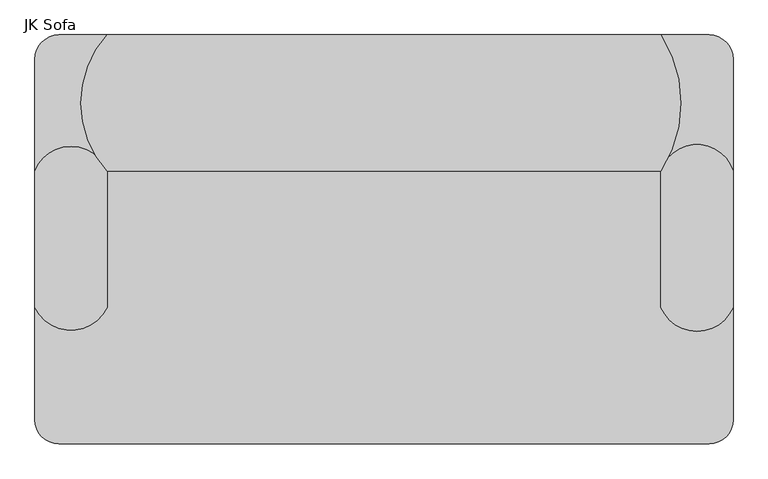
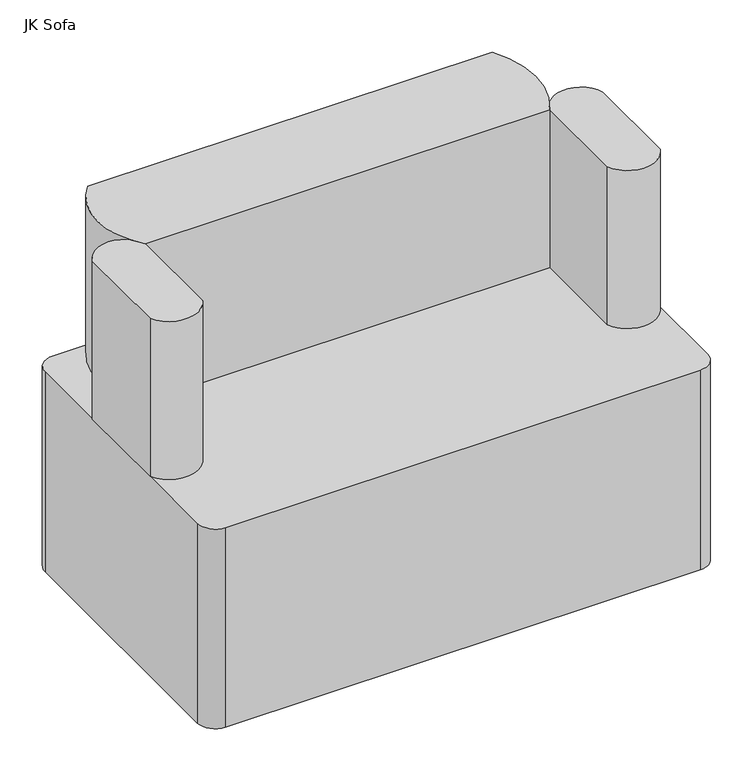
"""IFC4 building model written with IfcOpenShell, lengths in millimetres: furniture geometry, JK Sofa : 58 x 34 loveseat."""

from ifc_helpers import new_model, si_unit, point, frame, frame_2d, origin, origin_with_axes, place, context, project, spatial, polyline, circle_curve, trimmed, segment, composite_curve, outline, extrude, source, transform, mapped, element, save


def jk_sofa_d9d3c8d7(model_context):
    return source(origin(), model_context, "Body", "SweptSolid", [
        extrude(outline(composite_curve([segment(polyline([(522.2573665, 177.4788629), (-646.1426335, 177.4788629)]), True, "CONTINUOUS"), segment(trimmed(circle_curve(frame_2d((-486.5613896, 321.4121962)), 214.9022518), [point((-646.1426335, 177.4788629))], [point((-646.1426335, 465.3455296))], False, "CARTESIAN"), True, "CONTINUOUS"), segment(polyline([(-646.1426335, 465.3455296), (522.2573665, 465.3455296)]), True, "CONTINUOUS"), segment(trimmed(circle_curve(frame_2d((296.8181811, 321.4121962)), 267.4689342), [point((522.2573665, 465.3455296))], [point((522.2573665, 177.4788629))], False, "CARTESIAN"), True, "CONTINUOUS")], self_intersect=False)), frame((0.0, 0.0, 609.6), z_axis=(0.0, 0.0, 1.0), x_axis=(1.0, 0.0, 0.0)), (0.0, 0.0, 1.0), 482.6),
        extrude(outline(composite_curve([segment(polyline([(-798.5426335, -110.3878038), (-798.5426335, 177.4788629)]), True, "CONTINUOUS"), segment(trimmed(circle_curve(frame_2d((-722.3426335, 147.712096)), 81.8077039), [point((-798.5426335, 177.4788629))], [point((-646.1426335, 177.4788629))], False, "CARTESIAN"), True, "CONTINUOUS"), segment(polyline([(-646.1426335, 177.4788629), (-646.1426335, -110.3878038)]), True, "CONTINUOUS"), segment(trimmed(circle_curve(frame_2d((-722.3426335, -73.3296897)), 84.733369), [point((-646.1426335, -110.3878038))], [point((-798.5426335, -110.3878038))], False, "CARTESIAN"), True, "CONTINUOUS")], self_intersect=False)), frame((0.0, 0.0, 609.6), z_axis=(0.0, 0.0, 1.0), x_axis=(1.0, 0.0, 0.0)), (0.0, 0.0, 1.0), 482.6),
        extrude(outline(composite_curve([segment(polyline([(674.6573665, 177.4788629), (674.6573665, -110.3878038)]), True, "CONTINUOUS"), segment(trimmed(circle_curve(frame_2d((598.4573665, -78.2408831)), 82.7034734), [point((674.6573665, -110.3878038))], [point((522.2573665, -110.3878038))], False, "CARTESIAN"), True, "CONTINUOUS"), segment(polyline([(522.2573665, -110.3878038), (522.2573665, 177.4788629)]), True, "CONTINUOUS"), segment(trimmed(circle_curve(frame_2d((598.4573665, 153.7481356)), 79.809695), [point((522.2573665, 177.4788629))], [point((674.6573665, 177.4788629))], False, "CARTESIAN"), True, "CONTINUOUS")], self_intersect=False)), frame((0.0, 0.0, 609.6), z_axis=(0.0, 0.0, 1.0), x_axis=(1.0, 0.0, 0.0)), (0.0, 0.0, 1.0), 482.6),
        extrude(outline(composite_curve([segment(trimmed(circle_curve(frame_2d((623.8573665, 414.5455296)), 50.8), [point((623.8573665, 465.3455296))], [point((674.6573665, 414.5455296))], False, "CARTESIAN"), True, "CONTINUOUS"), segment(polyline([(674.6573665, 414.5455296), (674.6573665, -347.4544704)]), True, "CONTINUOUS"), segment(trimmed(circle_curve(frame_2d((623.8573665, -347.4544704)), 50.8), [point((674.6573665, -347.4544704))], [point((623.8573665, -398.2544704))], False, "CARTESIAN"), True, "CONTINUOUS"), segment(polyline([(623.8573665, -398.2544704), (-747.7426335, -398.2544704)]), True, "CONTINUOUS"), segment(trimmed(circle_curve(frame_2d((-747.7426335, -347.4544704)), 50.8), [point((-747.7426335, -398.2544704))], [point((-798.5426335, -347.4544704))], False, "CARTESIAN"), True, "CONTINUOUS"), segment(polyline([(-798.5426335, -347.4544704), (-798.5426335, 414.5455296)]), True, "CONTINUOUS"), segment(trimmed(circle_curve(frame_2d((-747.7426335, 414.5455296)), 50.8), [point((-798.5426335, 414.5455296))], [point((-747.7426335, 465.3455296))], False, "CARTESIAN"), True, "CONTINUOUS"), segment(polyline([(-747.7426335, 465.3455296), (623.8573665, 465.3455296)]), True, "CONTINUOUS")], self_intersect=False)), origin_with_axes(), (0.0, 0.0, 1.0), 609.6),
    ])


if __name__ == "__main__":
    model = new_model("IFC4")
    model_context = context("Model", 3, world=origin())
    ifc_project = project(units=[si_unit("LENGTHUNIT", "METRE", prefix="MILLI")], contexts=[model_context])
    site = spatial("IfcSite", under=ifc_project)
    building = spatial("IfcBuilding", under=site)
    placement = place(None, origin())
    jk_sofa_shape = jk_sofa_d9d3c8d7(model_context)
    element("IfcFurniture", 1, ObjectType="JK Sofa : 58 x 34 loveseat", at=placement, inside=building, context=model_context, shape_type="MappedRepresentation", body=[
        mapped(jk_sofa_shape, transform((0.0, 0.0, 0.0), x_axis=(1.0, 0.0, 0.0), y_axis=(0.0, 1.0, 0.0), z_axis=(0.0, 0.0, 1.0))),
    ])
    save(model, "model.ifc")

# Revit data of these elements
# Type "JK Sofa : 58 x 34 loveseat"
#   Width = 4' - 10"
#   Seat Height = 2' - 0"
#   Depth = 2' - 10"
#   Corner Radius = 0' - 2"
#   Back Height = 3' - 7"
#   Arm Width = 0' - 6"
#   Status [instance default] = none
#   Default Elevation = 0
